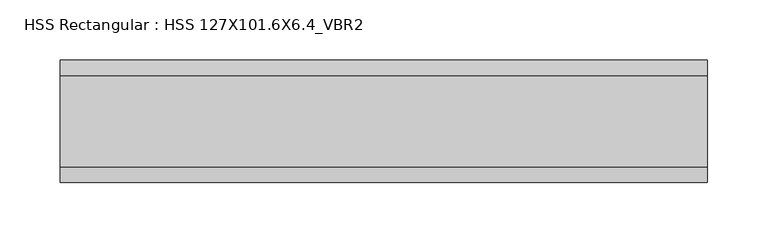
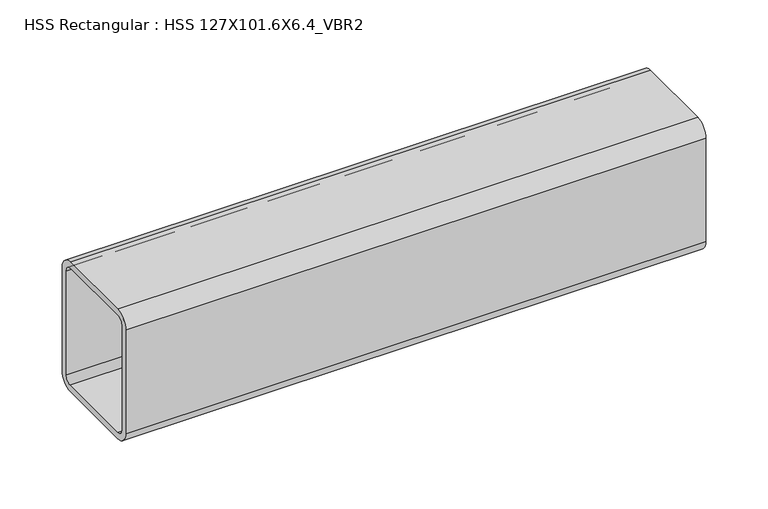
"""IFC4 building model written with IfcOpenShell, lengths in millimetres: member geometry, HSS Rectangular : HSS 127X101.6X6.4_VBR2."""

from ifc_helpers import new_model, si_unit, point, frame, frame_2d, origin, place, context, project, spatial, polyline, circle_curve, trimmed, segment, composite_curve, outline, extrude, source, transform, mapped, element, save


def hss_rectangular_hss_127x101_6x6_4_vbr2_996c7ac0(model_context):
    return source(origin(), model_context, "Body", "SweptSolid", [
        extrude(outline(composite_curve([segment(polyline([(50.8, 50.8), (50.8, -50.8)]), True, "CONTINUOUS"), segment(trimmed(circle_curve(frame_2d((38.1, -50.8)), 12.7), [point((50.8, -50.8))], [point((38.1, -63.5))], False, "CARTESIAN"), True, "CONTINUOUS"), segment(polyline([(38.1, -63.5), (-38.1, -63.5)]), True, "CONTINUOUS"), segment(trimmed(circle_curve(frame_2d((-38.1, -50.8)), 12.7), [point((-38.1, -63.5))], [point((-50.8, -50.8))], False, "CARTESIAN"), True, "CONTINUOUS"), segment(polyline([(-50.8, -50.8), (-50.8, 50.8)]), True, "CONTINUOUS"), segment(trimmed(circle_curve(frame_2d((-38.1, 50.8)), 12.7), [point((-50.8, 50.8))], [point((-38.1, 63.5))], False, "CARTESIAN"), True, "CONTINUOUS"), segment(polyline([(-38.1, 63.5), (38.1, 63.5)]), True, "CONTINUOUS"), segment(trimmed(circle_curve(frame_2d((38.1, 50.8)), 12.7), [point((38.1, 63.5))], [point((50.8, 50.8))], False, "CARTESIAN"), True, "CONTINUOUS")], self_intersect=False), holes=[composite_curve([segment(trimmed(circle_curve(frame_2d((-38.1, 50.8)), 6.35), [point((-38.1, 57.15))], [point((-44.45, 50.8))], True, "CARTESIAN"), True, "CONTINUOUS"), segment(polyline([(-44.45, 50.8), (-44.45, -50.8)]), True, "CONTINUOUS"), segment(trimmed(circle_curve(frame_2d((-38.1, -50.8)), 6.35), [point((-44.45, -50.8))], [point((-38.1, -57.15))], True, "CARTESIAN"), True, "CONTINUOUS"), segment(polyline([(-38.1, -57.15), (38.1, -57.15)]), True, "CONTINUOUS"), segment(trimmed(circle_curve(frame_2d((38.1, -50.8)), 6.35), [point((38.1, -57.15))], [point((44.45, -50.8))], True, "CARTESIAN"), True, "CONTINUOUS"), segment(polyline([(44.45, -50.8), (44.45, 50.8)]), True, "CONTINUOUS"), segment(trimmed(circle_curve(frame_2d((38.1, 50.8)), 6.35), [point((44.45, 50.8))], [point((38.1, 57.15))], True, "CARTESIAN"), True, "CONTINUOUS"), segment(polyline([(38.1, 57.15), (-38.1, 57.15)]), True, "CONTINUOUS")], self_intersect=False)]), frame((-251.8896058, 0.0, 0.0), z_axis=(1.0, 0.0, 0.0), x_axis=(0.0, 1.0, 0.0)), (0.0, 0.0, 1.0), 537.1503652),
    ])


if __name__ == "__main__":
    model = new_model("IFC4")
    model_context = context("Model", 3, world=origin())
    ifc_project = project(units=[si_unit("LENGTHUNIT", "METRE", prefix="MILLI")], contexts=[model_context])
    site = spatial("IfcSite", under=ifc_project)
    building = spatial("IfcBuilding", under=site)
    placement = place(None, origin())
    hss_rectangular_hss_127x101_6x6_4_vbr2_shape = hss_rectangular_hss_127x101_6x6_4_vbr2_996c7ac0(model_context)
    element("IfcMember", 1, ObjectType="HSS Rectangular : HSS 127X101.6X6.4_VBR2", at=placement, inside=building, context=model_context, shape_type="MappedRepresentation", body=[
        mapped(hss_rectangular_hss_127x101_6x6_4_vbr2_shape, transform((0.0, 0.0, 0.0), x_axis=(1.0, 0.0, 0.0), y_axis=(0.0, 1.0, 0.0), z_axis=(0.0, 0.0, 1.0))),
    ])
    save(model, "model.ifc")

# Revit data of these elements
# Type "HSS Rectangular : HSS 127X101.6X6.4_VBR2"
#   Section Name Key = "HSS5X4X1/4"
#   Assembly Code = "B10"
#   Width = 10.16 cm
#   Wall Nominal Thickness = 0.635 cm
#   Wall Design Thickness = 0.5918 cm
#   Torsional Moment of Inertia = 749.217 cm⁴
#   Torsional Modulus = 136.34 cm³
#   Section Area = 24.7741 cm²
#   Plastic Modulus weak axis = 91.2759 cm³
#   Plastic Modulus strong axis = 106.352 cm³
#   Perimeter = 0.435254 m²/m
#   Outer Fillet = 1.27 cm
#   Nominal Weight = 20.7004 kgf/m
#   Moment of Inertia weak axis = 393.755 cm⁴
#   Moment of Inertia strong axis = 557.75 cm⁴
#   Inner Fillet = 0.635 cm
#   Height = 12.7 cm
#   Elastic Modulus weak axis = 77.5108 cm³
#   Elastic Modulus strong axis = 87.6708 cm³
#   Centroid Vertical = 6.35 cm
#   Centroid Horizontal = 5.08 cm
#   Length [instance default] = 1524 mm
#   Structural Material [instance default] = Steel ASTM A500, Grade C, Rectangular and Square
#   Principal Axes Angle = 0
# Element 1 (IfcMember, "HSS Rectangular : HSS 127X101.6X6.4_VBR2")
#   Materials on its faces: "Steel ASTM A500, Grade C, Rectangular and Square"
# Materials
#   "Steel ASTM A500, Grade C, Rectangular and Square": class "Metal", colour RGB 120 120 120, transparency 0, Description = "Carbon steel", Cost = 0
